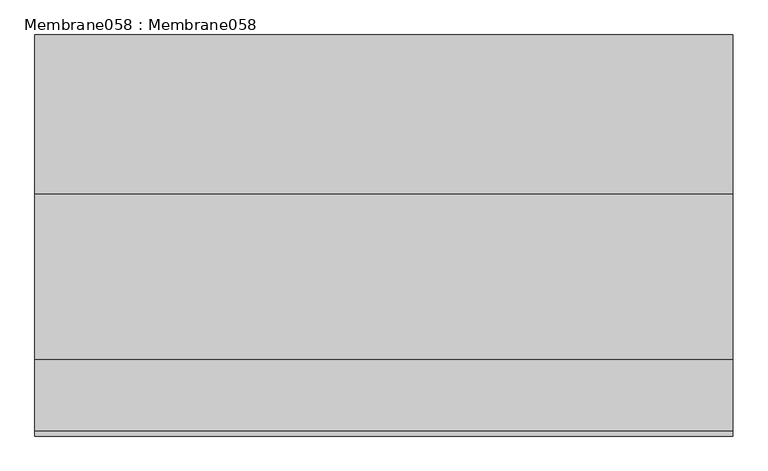
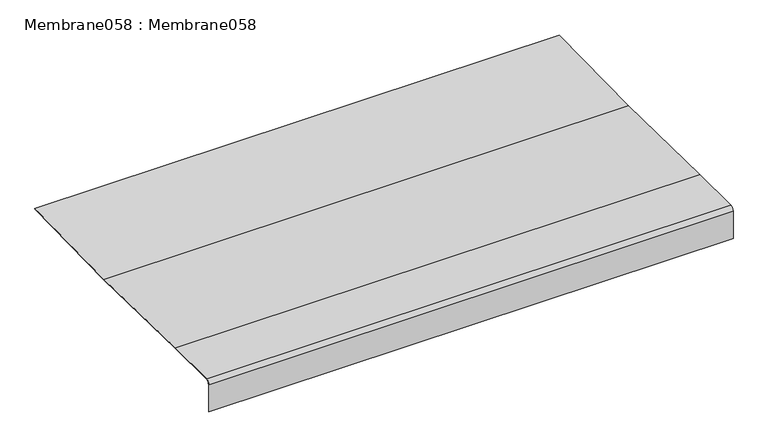
"""IFC4 building model written with IfcOpenShell, lengths in millimetres: proxy geometry, Membrane058 : Membrane058."""

import ifcopenshell
import ifcopenshell.guid

model = None  # the IFC model being written
_history = None  # IfcOwnerHistory: only IFC2X3 demands one
_inside = {}  # id of a spatial element -> (the spatial element, [elements in it])
_under = {}  # id of a project, library or spatial element -> (it, [spatial elements below it])
_declared = {}  # id of a project -> (the project, [libraries it declares])
_typed = {}  # id of a type object -> (the type object, [elements of that type])
_made_of = {}  # id of a material, layer set ... -> (it, [elements and type objects made of it])


def new_model(schema):
    """Start an empty IFC model of exactly this schema.

    Asked for "IFC4X3", IfcOpenShell would pick the latest addendum, in which some entities
    have other attributes; the version numbers below select the first issue.
    IFC2X3 requires an IfcOwnerHistory on every rooted entity: one is made here for all.
    """
    global model, _history
    if schema == "IFC4X3":
        model = ifcopenshell.file(schema_version=(4, 3, 0, 0))
    else:
        model = ifcopenshell.file(schema=schema)
    _inside.clear()
    _under.clear()
    _declared.clear()
    _typed.clear()
    _made_of.clear()
    _history = None
    if model.schema == "IFC2X3":
        org = make("IfcOrganization", Name="unknown")
        user = make(
            "IfcPersonAndOrganization",
            ThePerson=make("IfcPerson", FamilyName="unknown"),
            TheOrganization=org,
        )
        app = make(
            "IfcApplication",
            ApplicationDeveloper=org,
            Version="unknown",
            ApplicationFullName="unknown",
            ApplicationIdentifier="unknown",
        )
        _history = make(
            "IfcOwnerHistory",
            OwningUser=user,
            OwningApplication=app,
            ChangeAction="ADDED",
            CreationDate=0,
        )
    return model


def make(cls, **values):
    """One entity of the class cls with the attributes given. An attribute that is None is left unset."""
    return model.create_entity(
        cls, **{name: value for name, value in values.items() if value is not None}
    )


def rooted(cls, **values):
    """An entity with a GlobalId (a new one), such as an element, a storey or a relation."""
    return make(cls, GlobalId=ifcopenshell.guid.new(), OwnerHistory=_history, **values)


def si_unit(unit_type, name, prefix=None):
    """IfcSIUnit, for example si_unit("LENGTHUNIT", "METRE", prefix="MILLI")."""
    return make("IfcSIUnit", UnitType=unit_type, Prefix=prefix, Name=name)


def assignment(units):
    """IfcUnitAssignment: the units of a project."""
    return None if units is None else make("IfcUnitAssignment", Units=units)


def point(xyz):
    """IfcCartesianPoint."""
    return None if xyz is None else make("IfcCartesianPoint", Coordinates=xyz)


def direction(xyz):
    """IfcDirection."""
    return None if xyz is None else make("IfcDirection", DirectionRatios=xyz)


def frame(location, z_axis=None, x_axis=None):
    """IfcAxis2Placement3D, a coordinate frame: its origin and axes. An axis left out is left unset."""
    return make(
        "IfcAxis2Placement3D",
        Location=point(location),
        Axis=direction(z_axis),
        RefDirection=direction(x_axis),
    )


def frame_2d(location, x_axis=None):
    """IfcAxis2Placement2D, a coordinate frame in the plane: its origin and x axis."""
    return make(
        "IfcAxis2Placement2D", Location=point(location), RefDirection=direction(x_axis)
    )


def origin():
    """The frame at (0, 0, 0) with its axes left unset."""
    return frame((0.0, 0.0, 0.0))


def place(relative_to, where):
    """IfcLocalPlacement: puts the frame where relative to a parent placement (None: the world)."""
    return make(
        "IfcLocalPlacement", PlacementRelTo=relative_to, RelativePlacement=where
    )


def context(
    kind, dimensions, precision=None, world=None, true_north=None, identifier=None
):
    """IfcGeometricRepresentationContext, for example the 3D "Model" context."""
    return make(
        "IfcGeometricRepresentationContext",
        ContextIdentifier=identifier,
        ContextType=kind,
        CoordinateSpaceDimension=dimensions,
        Precision=precision,
        WorldCoordinateSystem=world,
        TrueNorth=true_north,
    )


def project(units=None, contexts=None):
    """IfcProject with its units and contexts."""
    return rooted(
        "IfcProject",
        Name="project",
        RepresentationContexts=contexts,
        UnitsInContext=assignment(units),
    )


def spatial(cls, under=None, at=None, **own):
    """A site, building, storey or space (cls), placed at a placement, below another one or the project."""
    s = rooted(cls, ObjectPlacement=at, **own)
    if under is not None:
        _under.setdefault(under.id(), (under, []))[1].append(s)
    return s


def polyline(points):
    """IfcPolyline through the points."""
    return make("IfcPolyline", Points=[point(p) for p in points])


def circle_curve(where, radius):
    """IfcCircle in the frame where."""
    return make("IfcCircle", Position=where, Radius=radius)


def trimmed(basis, trim1, trim2, sense, master):
    """IfcTrimmedCurve: the piece of a basis curve between two trims."""
    return make(
        "IfcTrimmedCurve",
        BasisCurve=basis,
        Trim1=trim1,
        Trim2=trim2,
        SenseAgreement=sense,
        MasterRepresentation=master,
    )


def segment(curve, same_sense, transition):
    """IfcCompositeCurveSegment."""
    return make(
        "IfcCompositeCurveSegment",
        Transition=transition,
        SameSense=same_sense,
        ParentCurve=curve,
    )


def composite_curve(segments, self_intersect=None):
    """IfcCompositeCurve: segments joined end to end."""
    return make("IfcCompositeCurve", Segments=segments, SelfIntersect=self_intersect)


def outline(outer, holes=None, kind="AREA"):
    """IfcArbitraryClosedProfileDef: a profile drawn as a closed curve; with holes, ...WithVoids."""
    if holes is None:
        return make("IfcArbitraryClosedProfileDef", ProfileType=kind, OuterCurve=outer)
    return make(
        "IfcArbitraryProfileDefWithVoids",
        ProfileType=kind,
        OuterCurve=outer,
        InnerCurves=holes,
    )


def extrude(swept, where, along, depth):
    """IfcExtrudedAreaSolid: the profile swept, set in the frame where, extruded along a direction by depth."""
    return make(
        "IfcExtrudedAreaSolid",
        SweptArea=swept,
        Position=where,
        ExtrudedDirection=direction(along),
        Depth=depth,
    )


def shape(context_of_items, identifier, shape_type, items):
    """IfcShapeRepresentation: the items that make up one representation, for example the "Body"."""
    return make(
        "IfcShapeRepresentation",
        ContextOfItems=context_of_items,
        RepresentationIdentifier=identifier,
        RepresentationType=shape_type,
        Items=items,
    )


def source(mapping_origin, context_of_items, identifier, shape_type, items):
    """IfcRepresentationMap: a shape defined once, which mapped items show again and again."""
    return make(
        "IfcRepresentationMap",
        MappingOrigin=mapping_origin,
        MappedRepresentation=shape(context_of_items, identifier, shape_type, items),
    )


def transform(
    local_origin,
    x_axis=None,
    y_axis=None,
    z_axis=None,
    scale=None,
    scale2=None,
    scale3=None,
    uniform=True,
):
    """IfcCartesianTransformationOperator3D, or its non-uniform kind. x_axis, y_axis, z_axis: its Axis1, 2, 3."""
    if uniform:
        return make(
            "IfcCartesianTransformationOperator3D",
            Axis1=direction(x_axis),
            Axis2=direction(y_axis),
            LocalOrigin=point(local_origin),
            Scale=scale,
            Axis3=direction(z_axis),
        )
    return make(
        "IfcCartesianTransformationOperator3DnonUniform",
        Axis1=direction(x_axis),
        Axis2=direction(y_axis),
        LocalOrigin=point(local_origin),
        Scale=scale,
        Axis3=direction(z_axis),
        Scale2=scale2,
        Scale3=scale3,
    )


def mapped(mapping_source, mapping_target):
    """IfcMappedItem: shows the shape of a source again, moved by a transform."""
    return make(
        "IfcMappedItem", MappingSource=mapping_source, MappingTarget=mapping_target
    )


def made_of(thing, what):
    """Note that an element or type object is made of a material, layer set ...; save() writes the relation."""
    if what is not None:
        _made_of.setdefault(what.id(), (what, []))[1].append(thing)
    return thing


def element(
    cls,
    number,
    at=None,
    inside=None,
    cuts=None,
    type_object=None,
    material=None,
    context=None,
    identifier="Body",
    shape_type=None,
    held_by="IfcProductDefinitionShape",
    body=None,
    shapes=None,
    **own,
):
    """One element of the class cls, such as IfcWall. Its Tag is "e" and its number.

    at: its placement. inside: the storey or other place that contains it. cuts: it is an
    opening in that element (IfcRelVoidsElement). A single representation is given by context,
    identifier, shape_type and body (its items); several are given by shapes. held_by: the class
    of the entity that holds the representations. save() writes the other relations.
    """
    e = rooted(cls, Tag="e%d" % number, ObjectPlacement=at, **own)
    if body is not None:
        shapes = [shape(context, identifier, shape_type, body)]
    if shapes is not None:
        e.Representation = make(held_by, Representations=shapes)
    if inside is not None:
        _inside.setdefault(inside.id(), (inside, []))[1].append(e)
    if cuts is not None:
        rooted(
            "IfcRelVoidsElement", RelatingBuildingElement=cuts, RelatedOpeningElement=e
        )
    if type_object is not None:
        _typed.setdefault(type_object.id(), (type_object, []))[1].append(e)
    return made_of(e, material)


def aggregate(whole, parts):
    """IfcRelAggregates: a whole, such as a stair, and the parts it consists of."""
    return rooted("IfcRelAggregates", RelatingObject=whole, RelatedObjects=parts)


def save(model, path):
    """Write the relations noted so far, then the file.

    IfcRelAggregates (storeys below a building ...), IfcRelContainedInSpatialStructure (elements
    in a storey), IfcRelDefinesByType, IfcRelAssociatesMaterial and IfcRelDeclares: one each for
    every whole, place, type object, material and project.
    """
    for whole, parts in _under.values():
        aggregate(whole, parts)
    for where, things in _inside.values():
        rooted(
            "IfcRelContainedInSpatialStructure",
            RelatedElements=things,
            RelatingStructure=where,
        )
    for kind, things in _typed.values():
        rooted("IfcRelDefinesByType", RelatedObjects=things, RelatingType=kind)
    for what, things in _made_of.values():
        rooted("IfcRelAssociatesMaterial", RelatedObjects=things, RelatingMaterial=what)
    for by, libraries in _declared.values():
        rooted("IfcRelDeclares", RelatingContext=by, RelatedDefinitions=libraries)
    model.write(path)


def membrane058_membrane058_c6d29274(model_context):
    return source(origin(), model_context, "Body", "SweptSolid", [
        extrude(outline(composite_curve([segment(polyline([(109.5960262, 0.0), (109.5960262, -2.0), (0.0, -2.0)]), True, "CONTINUOUS"), segment(trimmed(circle_curve(frame_2d((0.0, 13.0)), 15.0), [point((0.0, -2.0))], [point((-15.0, 13.0))], False, "CARTESIAN"), True, "CONTINUOUS"), segment(polyline([(-15.0, 13.0), (-15.0, 218.6766472), (-4.1647274, 692.2700153), (-14.0116379, 1147.1048908), (-12.0121064, 1147.1481795), (-2.1642322, 692.2687862), (-13.0, 218.6537713), (-13.0, 13.0)]), True, "CONTINUOUS"), segment(trimmed(circle_curve(frame_2d((0.0, 13.0)), 13.0), [point((-13.0, 13.0))], [point((0.0, 0.0))], True, "CARTESIAN"), True, "CONTINUOUS"), segment(polyline([(0.0, 0.0), (109.5960262, 0.0)]), True, "CONTINUOUS")], self_intersect=False)), frame((12383.0178845, -5570.4475281, 40220.1581398), z_axis=(1.0, 0.0, -1.65992950796479e-11), x_axis=(-1.65992950796479e-11, 0.0, -1.0)), (0.0, 0.0, 1.0), 2000.0),
    ])


if __name__ == "__main__":
    model = new_model("IFC4")
    model_context = context("Model", 3, world=origin())
    ifc_project = project(units=[si_unit("LENGTHUNIT", "METRE", prefix="MILLI")], contexts=[model_context])
    site = spatial("IfcSite", under=ifc_project)
    building = spatial("IfcBuilding", under=site)
    placement = place(None, origin())
    membrane058_membrane058_shape = membrane058_membrane058_c6d29274(model_context)
    element("IfcBuildingElementProxy", 1, Name="Membrane058 : Membrane058", ObjectType="Membrane058 : Membrane058", at=placement, inside=building, context=model_context, shape_type="MappedRepresentation", body=[
        mapped(membrane058_membrane058_shape, transform((0.0, 0.0, 0.0), x_axis=(1.0, 0.0, 0.0), y_axis=(0.0, 1.0, 0.0), z_axis=(0.0, 0.0, 1.0))),
    ])
    save(model, "model.ifc")

# Revit data of these elements
# Type "Membrane058 : Membrane058"
#   NameOverride = "Membrane058"
# Element 1 (IfcBuildingElementProxy, "Membrane058 : Membrane058")
#   Materials on its faces: "THREE PLY BUILT UP ROOF MEMBRANE"
# Materials
#   "THREE PLY BUILT UP ROOF MEMBRANE": class "Unassigned", colour RGB 63 63 63, transparency 0
